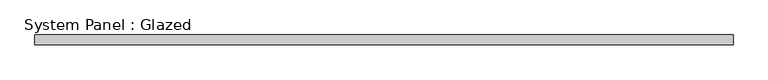
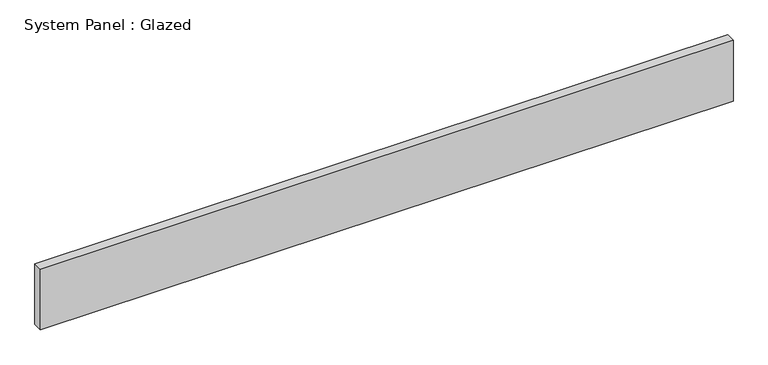
"""IFC4 building model written with IfcOpenShell, lengths in millimetres: plate geometry, System Panel : Glazed."""

import ifcopenshell
import ifcopenshell.guid

model = None  # the IFC model being written
_history = None  # IfcOwnerHistory: only IFC2X3 demands one
_inside = {}  # id of a spatial element -> (the spatial element, [elements in it])
_under = {}  # id of a project, library or spatial element -> (it, [spatial elements below it])
_declared = {}  # id of a project -> (the project, [libraries it declares])
_typed = {}  # id of a type object -> (the type object, [elements of that type])
_made_of = {}  # id of a material, layer set ... -> (it, [elements and type objects made of it])


def new_model(schema):
    """Start an empty IFC model of exactly this schema.

    Asked for "IFC4X3", IfcOpenShell would pick the latest addendum, in which some entities
    have other attributes; the version numbers below select the first issue.
    IFC2X3 requires an IfcOwnerHistory on every rooted entity: one is made here for all.
    """
    global model, _history
    if schema == "IFC4X3":
        model = ifcopenshell.file(schema_version=(4, 3, 0, 0))
    else:
        model = ifcopenshell.file(schema=schema)
    _inside.clear()
    _under.clear()
    _declared.clear()
    _typed.clear()
    _made_of.clear()
    _history = None
    if model.schema == "IFC2X3":
        org = make("IfcOrganization", Name="unknown")
        user = make(
            "IfcPersonAndOrganization",
            ThePerson=make("IfcPerson", FamilyName="unknown"),
            TheOrganization=org,
        )
        app = make(
            "IfcApplication",
            ApplicationDeveloper=org,
            Version="unknown",
            ApplicationFullName="unknown",
            ApplicationIdentifier="unknown",
        )
        _history = make(
            "IfcOwnerHistory",
            OwningUser=user,
            OwningApplication=app,
            ChangeAction="ADDED",
            CreationDate=0,
        )
    return model


def make(cls, **values):
    """One entity of the class cls with the attributes given. An attribute that is None is left unset."""
    return model.create_entity(
        cls, **{name: value for name, value in values.items() if value is not None}
    )


def rooted(cls, **values):
    """An entity with a GlobalId (a new one), such as an element, a storey or a relation."""
    return make(cls, GlobalId=ifcopenshell.guid.new(), OwnerHistory=_history, **values)


def si_unit(unit_type, name, prefix=None):
    """IfcSIUnit, for example si_unit("LENGTHUNIT", "METRE", prefix="MILLI")."""
    return make("IfcSIUnit", UnitType=unit_type, Prefix=prefix, Name=name)


def assignment(units):
    """IfcUnitAssignment: the units of a project."""
    return None if units is None else make("IfcUnitAssignment", Units=units)


def point(xyz):
    """IfcCartesianPoint."""
    return None if xyz is None else make("IfcCartesianPoint", Coordinates=xyz)


def direction(xyz):
    """IfcDirection."""
    return None if xyz is None else make("IfcDirection", DirectionRatios=xyz)


def frame(location, z_axis=None, x_axis=None):
    """IfcAxis2Placement3D, a coordinate frame: its origin and axes. An axis left out is left unset."""
    return make(
        "IfcAxis2Placement3D",
        Location=point(location),
        Axis=direction(z_axis),
        RefDirection=direction(x_axis),
    )


def origin():
    """The frame at (0, 0, 0) with its axes left unset."""
    return frame((0.0, 0.0, 0.0))


def origin_with_axes():
    """The frame at (0, 0, 0) with the z axis (0, 0, 1) and the x axis (1, 0, 0) written out."""
    return frame((0.0, 0.0, 0.0), z_axis=(0.0, 0.0, 1.0), x_axis=(1.0, 0.0, 0.0))


def place(relative_to, where):
    """IfcLocalPlacement: puts the frame where relative to a parent placement (None: the world)."""
    return make(
        "IfcLocalPlacement", PlacementRelTo=relative_to, RelativePlacement=where
    )


def context(
    kind, dimensions, precision=None, world=None, true_north=None, identifier=None
):
    """IfcGeometricRepresentationContext, for example the 3D "Model" context."""
    return make(
        "IfcGeometricRepresentationContext",
        ContextIdentifier=identifier,
        ContextType=kind,
        CoordinateSpaceDimension=dimensions,
        Precision=precision,
        WorldCoordinateSystem=world,
        TrueNorth=true_north,
    )


def project(units=None, contexts=None):
    """IfcProject with its units and contexts."""
    return rooted(
        "IfcProject",
        Name="project",
        RepresentationContexts=contexts,
        UnitsInContext=assignment(units),
    )


def spatial(cls, under=None, at=None, **own):
    """A site, building, storey or space (cls), placed at a placement, below another one or the project."""
    s = rooted(cls, ObjectPlacement=at, **own)
    if under is not None:
        _under.setdefault(under.id(), (under, []))[1].append(s)
    return s


def polyline(points):
    """IfcPolyline through the points."""
    return make("IfcPolyline", Points=[point(p) for p in points])


def outline(outer, holes=None, kind="AREA"):
    """IfcArbitraryClosedProfileDef: a profile drawn as a closed curve; with holes, ...WithVoids."""
    if holes is None:
        return make("IfcArbitraryClosedProfileDef", ProfileType=kind, OuterCurve=outer)
    return make(
        "IfcArbitraryProfileDefWithVoids",
        ProfileType=kind,
        OuterCurve=outer,
        InnerCurves=holes,
    )


def extrude(swept, where, along, depth):
    """IfcExtrudedAreaSolid: the profile swept, set in the frame where, extruded along a direction by depth."""
    return make(
        "IfcExtrudedAreaSolid",
        SweptArea=swept,
        Position=where,
        ExtrudedDirection=direction(along),
        Depth=depth,
    )


def shape(context_of_items, identifier, shape_type, items):
    """IfcShapeRepresentation: the items that make up one representation, for example the "Body"."""
    return make(
        "IfcShapeRepresentation",
        ContextOfItems=context_of_items,
        RepresentationIdentifier=identifier,
        RepresentationType=shape_type,
        Items=items,
    )


def source(mapping_origin, context_of_items, identifier, shape_type, items):
    """IfcRepresentationMap: a shape defined once, which mapped items show again and again."""
    return make(
        "IfcRepresentationMap",
        MappingOrigin=mapping_origin,
        MappedRepresentation=shape(context_of_items, identifier, shape_type, items),
    )


def transform(
    local_origin,
    x_axis=None,
    y_axis=None,
    z_axis=None,
    scale=None,
    scale2=None,
    scale3=None,
    uniform=True,
):
    """IfcCartesianTransformationOperator3D, or its non-uniform kind. x_axis, y_axis, z_axis: its Axis1, 2, 3."""
    if uniform:
        return make(
            "IfcCartesianTransformationOperator3D",
            Axis1=direction(x_axis),
            Axis2=direction(y_axis),
            LocalOrigin=point(local_origin),
            Scale=scale,
            Axis3=direction(z_axis),
        )
    return make(
        "IfcCartesianTransformationOperator3DnonUniform",
        Axis1=direction(x_axis),
        Axis2=direction(y_axis),
        LocalOrigin=point(local_origin),
        Scale=scale,
        Axis3=direction(z_axis),
        Scale2=scale2,
        Scale3=scale3,
    )


def mapped(mapping_source, mapping_target):
    """IfcMappedItem: shows the shape of a source again, moved by a transform."""
    return make(
        "IfcMappedItem", MappingSource=mapping_source, MappingTarget=mapping_target
    )


def made_of(thing, what):
    """Note that an element or type object is made of a material, layer set ...; save() writes the relation."""
    if what is not None:
        _made_of.setdefault(what.id(), (what, []))[1].append(thing)
    return thing


def element(
    cls,
    number,
    at=None,
    inside=None,
    cuts=None,
    type_object=None,
    material=None,
    context=None,
    identifier="Body",
    shape_type=None,
    held_by="IfcProductDefinitionShape",
    body=None,
    shapes=None,
    **own,
):
    """One element of the class cls, such as IfcWall. Its Tag is "e" and its number.

    at: its placement. inside: the storey or other place that contains it. cuts: it is an
    opening in that element (IfcRelVoidsElement). A single representation is given by context,
    identifier, shape_type and body (its items); several are given by shapes. held_by: the class
    of the entity that holds the representations. save() writes the other relations.
    """
    e = rooted(cls, Tag="e%d" % number, ObjectPlacement=at, **own)
    if body is not None:
        shapes = [shape(context, identifier, shape_type, body)]
    if shapes is not None:
        e.Representation = make(held_by, Representations=shapes)
    if inside is not None:
        _inside.setdefault(inside.id(), (inside, []))[1].append(e)
    if cuts is not None:
        rooted(
            "IfcRelVoidsElement", RelatingBuildingElement=cuts, RelatedOpeningElement=e
        )
    if type_object is not None:
        _typed.setdefault(type_object.id(), (type_object, []))[1].append(e)
    return made_of(e, material)


def aggregate(whole, parts):
    """IfcRelAggregates: a whole, such as a stair, and the parts it consists of."""
    return rooted("IfcRelAggregates", RelatingObject=whole, RelatedObjects=parts)


def save(model, path):
    """Write the relations noted so far, then the file.

    IfcRelAggregates (storeys below a building ...), IfcRelContainedInSpatialStructure (elements
    in a storey), IfcRelDefinesByType, IfcRelAssociatesMaterial and IfcRelDeclares: one each for
    every whole, place, type object, material and project.
    """
    for whole, parts in _under.values():
        aggregate(whole, parts)
    for where, things in _inside.values():
        rooted(
            "IfcRelContainedInSpatialStructure",
            RelatedElements=things,
            RelatingStructure=where,
        )
    for kind, things in _typed.values():
        rooted("IfcRelDefinesByType", RelatedObjects=things, RelatingType=kind)
    for what, things in _made_of.values():
        rooted("IfcRelAssociatesMaterial", RelatedObjects=things, RelatingMaterial=what)
    for by, libraries in _declared.values():
        rooted("IfcRelDeclares", RelatingContext=by, RelatedDefinitions=libraries)
    model.write(path)


def system_panel_glazed_f4345ae3(model_context):
    return source(origin(), model_context, "Body", "SweptSolid", [
        extrude(outline(polyline([(914.4, -44.45), (-914.4, -44.45), (-914.4, -19.05), (914.4, -19.05), (914.4, -44.45)])), origin_with_axes(), (0.0, 0.0, 1.0), 169.2731269),
    ])


if __name__ == "__main__":
    model = new_model("IFC4")
    model_context = context("Model", 3, world=origin())
    ifc_project = project(units=[si_unit("LENGTHUNIT", "METRE", prefix="MILLI")], contexts=[model_context])
    site = spatial("IfcSite", under=ifc_project)
    building = spatial("IfcBuilding", under=site)
    placement = place(None, origin())
    system_panel_glazed_shape = system_panel_glazed_f4345ae3(model_context)
    element("IfcPlate", 1, ObjectType="System Panel : Glazed", at=placement, inside=building, context=model_context, shape_type="MappedRepresentation", body=[
        mapped(system_panel_glazed_shape, transform((0.0, 0.0, 0.0), x_axis=(1.0, 0.0, 0.0), y_axis=(0.0, 1.0, 0.0), z_axis=(0.0, 0.0, 1.0))),
    ])
    save(model, "model.ifc")

# Revit data of these elements
# Type "System Panel : Glazed"
#   Construction Type Id = "GSP4R"
#   Analytic Construction = "1/8 in Pilkington single glazing"
#   Visual Light Transmittance = 0.9
#   Solar Heat Gain Coefficient = 0.86
#   Heat Transfer Coefficient (U) = 1.18115 BTU/(h·ft²·°F)
#   Define Thermal Properties by = 1
# Element 1 (IfcPlate, "System Panel : Glazed")
#   Materials on its faces: "Glass"
# Materials
#   "Glass": class "Glass", colour RGB 0 128 192, transparency 0.75, Description = "Soda Lime Glass", Cost = 0
